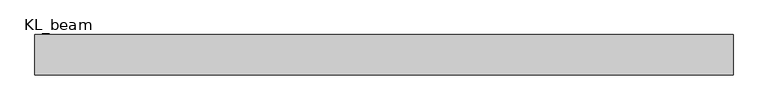
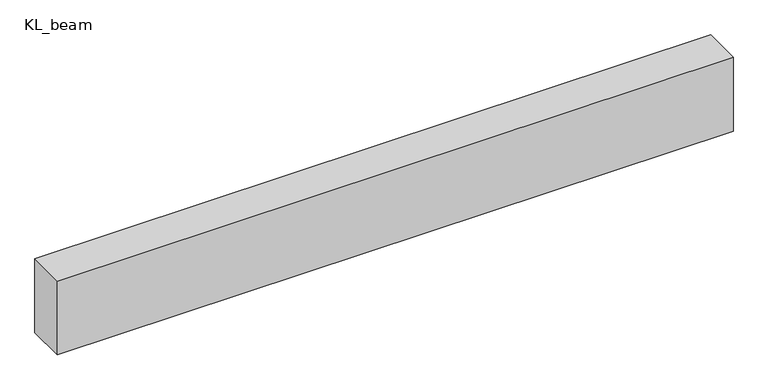
"""IFC4 building model written with IfcOpenShell, lengths in millimetres: beam geometry, 混凝土 - 矩形梁 : KL_beam."""

from ifc_helpers import new_model, si_unit, frame, origin, place, context, project, spatial, polyline, outline, extrude, source, transform, mapped, element, save


def kl_beam_cbf95bda(model_context):
    return source(origin(), model_context, "Body", "SweptSolid", [
        extrude(outline(polyline([(3460.0, 200.0), (3460.0, -200.0), (-3460.0, -200.0), (-3460.0, 200.0), (3460.0, 200.0)])), frame((0.0, 0.0, -400.0), z_axis=(0.0, 0.0, 1.0), x_axis=(1.0, 0.0, 0.0)), (0.0, 0.0, 1.0), 800.0),
    ])


if __name__ == "__main__":
    model = new_model("IFC4")
    model_context = context("Model", 3, world=origin())
    ifc_project = project(units=[si_unit("LENGTHUNIT", "METRE", prefix="MILLI")], contexts=[model_context])
    site = spatial("IfcSite", under=ifc_project)
    building = spatial("IfcBuilding", under=site)
    placement = place(None, origin())
    kl_beam_shape = kl_beam_cbf95bda(model_context)
    element("IfcBeam", 1, ObjectType="混凝土 - 矩形梁 : KL_beam", at=placement, inside=building, context=model_context, shape_type="MappedRepresentation", body=[
        mapped(kl_beam_shape, transform((0.0, 0.0, 0.0), x_axis=(1.0, 0.0, 0.0), y_axis=(0.0, 1.0, 0.0), z_axis=(0.0, 0.0, 1.0))),
    ])
    save(model, "model.ifc")

# Revit data of these elements
# Type "混凝土 - 矩形梁 : KL_beam"
#   Length [instance default] = 1524 mm
#   b = 400 mm
#   h = 800 mm
#   Structural Material [instance default] = 混凝土 - 现场浇注混凝土
#   Assembly Code = ""
# Element 1 (IfcBeam, "混凝土 - 矩形梁 : KL_beam")
#   Structural Material = none
# Materials
#   "混凝土 - 现场浇注混凝土": class "混凝土", colour RGB 192 192 192, transparency 0
